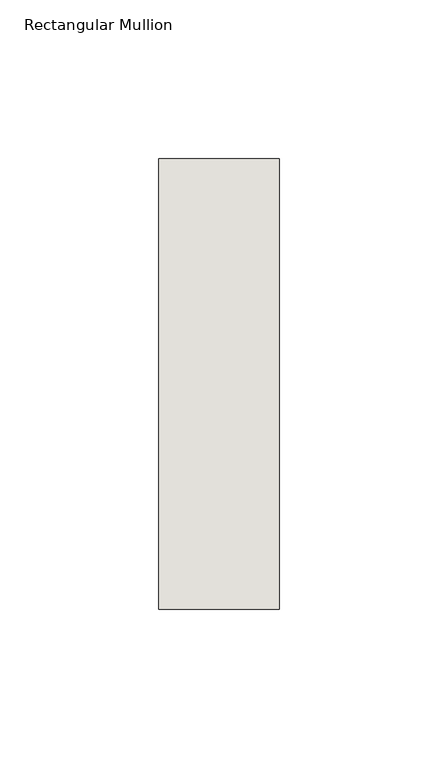
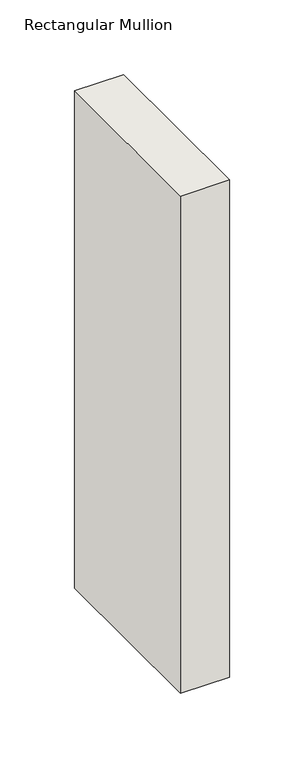
"""IFC4 building model written with IfcOpenShell, lengths in millimetres: wall geometry, Rectangular Mullion : NLRS_21_CWM_hsb-regel 38x142_gen_rsf."""

from ifc_helpers import new_model, si_unit, frame, origin, place, context, project, spatial, polyline, outline, extrude, source, transform, mapped, element, save


def rectangular_mullion_51268c3e(model_context):
    return source(origin(), model_context, "Body", "SweptSolid", [
        extrude(outline(polyline([(0.0, -71.0), (-38.0, -71.0), (-38.0, 71.0), (0.0, 71.0), (0.0, -71.0)])), frame((0.0, 0.0, -407.0), z_axis=(0.0, 0.0, 1.0), x_axis=(1.0, 0.0, 0.0)), (0.0, 0.0, 1.0), 407.0),
    ])


if __name__ == "__main__":
    model = new_model("IFC4")
    model_context = context("Model", 3, world=origin())
    ifc_project = project(units=[si_unit("LENGTHUNIT", "METRE", prefix="MILLI")], contexts=[model_context])
    site = spatial("IfcSite", under=ifc_project)
    building = spatial("IfcBuilding", under=site)
    placement = place(None, origin())
    rectangular_mullion_shape = rectangular_mullion_51268c3e(model_context)
    element("IfcWall", 1, ObjectType="Rectangular Mullion : NLRS_21_CWM_hsb-regel 38x142_gen_rsf", at=placement, inside=building, context=model_context, shape_type="MappedRepresentation", body=[
        mapped(rectangular_mullion_shape, transform((0.0, 0.0, 0.0), x_axis=(1.0, 0.0, 0.0), y_axis=(0.0, 1.0, 0.0), z_axis=(0.0, 0.0, 1.0))),
    ])
    save(model, "model.ifc")

# Revit data of these elements
# Type "Rectangular Mullion : NLRS_21_CWM_hsb-regel 38x142_gen_rsf"
#   Type IfcGUID = "07M7mRoiH1CR8m_RSKIwpF"
#   Assembly Code = "21.10"
#   IfcExportAs = "IfcWall"
#   built-in parameter 1007322 = 0.465879 (stored number, unit not read)
#   built-in parameter 1007321 = 0.062336 (stored number, unit not read)
#   built-in parameter 1007320 = 0.062336 (stored number, unit not read)
# Element 1 (IfcWall, "Rectangular Mullion : NLRS_21_CWM_hsb-regel 38x142_gen_rsf")
#   Materials on its faces: "NLRS_i2_hout naaldhout vuren_gen_rsf"
# Materials
#   "NLRS_i2_hout naaldhout vuren_gen_rsf": class "I - Hout", colour RGB 234 199 147, transparency 0, Keynote = "i2", Manufacturer = "Revit Standards Foundation", URL = "www.revitstandards.org", Description = "hout vuren", Cost = 0
